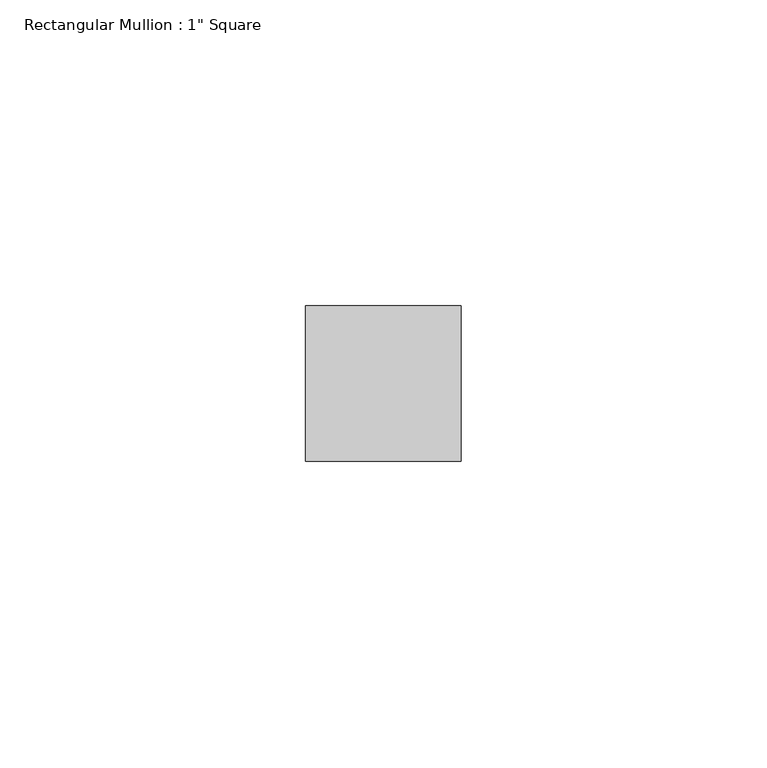
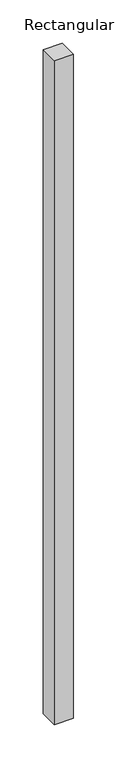
"""IFC4 building model written with IfcOpenShell, lengths in millimetres: member geometry."""

from ifc_helpers import new_model, si_unit, frame, origin, place, context, project, spatial, polyline, outline, extrude, source, transform, mapped, element, save


def member_bb84ead6(model_context):
    return source(origin(), model_context, "Body", "SweptSolid", [
        extrude(outline(polyline([(12.7, 12.7), (12.7, -12.7), (-12.7, -12.7), (-12.7, 12.7), (12.7, 12.7)])), frame((0.0, 0.0, -936.1811964), z_axis=(0.0, 0.0, 1.0), x_axis=(1.0, 0.0, 0.0)), (0.0, 0.0, 1.0), 936.1811964),
    ])


if __name__ == "__main__":
    model = new_model("IFC4")
    model_context = context("Model", 3, world=origin())
    ifc_project = project(units=[si_unit("LENGTHUNIT", "METRE", prefix="MILLI")], contexts=[model_context])
    site = spatial("IfcSite", under=ifc_project)
    building = spatial("IfcBuilding", under=site)
    placement = place(None, origin())
    member_shape = member_bb84ead6(model_context)
    element("IfcMember", 1, ObjectType="Rectangular Mullion : 1\" Square", at=placement, inside=building, context=model_context, shape_type="MappedRepresentation", body=[
        mapped(member_shape, transform((0.0, 0.0, 0.0), x_axis=(1.0, 0.0, 0.0), y_axis=(0.0, 1.0, 0.0), z_axis=(0.0, 0.0, 1.0))),
    ])
    save(model, "model.ifc")

# Revit data of these elements
# Type "Rectangular Mullion : 1\" Square"
#   built-in parameter 1007304 = 0.0833333 (stored number, unit not read)
#   built-in parameter 1007301 = 0.0416667 (stored number, unit not read)
#   built-in parameter 1007300 = 0.0416667 (stored number, unit not read)
# Element 1 (IfcMember, "Rectangular Mullion : 1\" Square")
#   Materials on its faces: "Metal - Aluminum"
# Materials
#   "Metal - Aluminum": class "Metal", colour RGB 247 247 247, transparency 0
